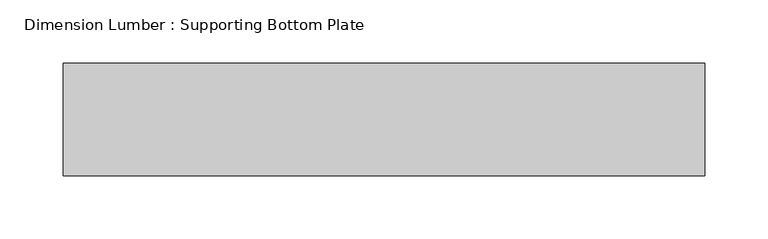
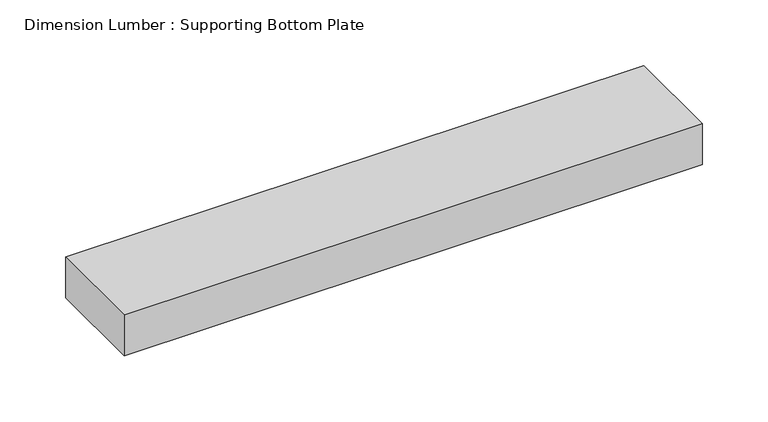
"""IFC4 building model written with IfcOpenShell, lengths in millimetres: beam geometry, Dimension Lumber : Supporting Bottom Plate."""

from ifc_helpers import new_model, si_unit, frame, origin, place, context, project, spatial, polyline, outline, extrude, source, transform, mapped, element, save


def dimension_lumber_supporting_bottom_plate_bde2bea7(model_context):
    return source(origin(), model_context, "Body", "SweptSolid", [
        extrude(outline(polyline([(-1203.025, 44.45), (-695.625, 44.45), (-695.625, -44.45), (-1203.025, -44.45), (-1203.025, 44.45)])), frame((0.0, 0.0, -19.05), z_axis=(0.0, 0.0, 1.0), x_axis=(1.0, 0.0, 0.0)), (0.0, 0.0, 1.0), 38.1),
    ])


if __name__ == "__main__":
    model = new_model("IFC4")
    model_context = context("Model", 3, world=origin())
    ifc_project = project(units=[si_unit("LENGTHUNIT", "METRE", prefix="MILLI")], contexts=[model_context])
    site = spatial("IfcSite", under=ifc_project)
    building = spatial("IfcBuilding", under=site)
    placement = place(None, origin())
    dimension_lumber_supporting_bottom_plate_shape = dimension_lumber_supporting_bottom_plate_bde2bea7(model_context)
    element("IfcBeam", 1, ObjectType="Dimension Lumber : Supporting Bottom Plate", at=placement, inside=building, context=model_context, shape_type="MappedRepresentation", body=[
        mapped(dimension_lumber_supporting_bottom_plate_shape, transform((0.0, 0.0, 0.0), x_axis=(1.0, 0.0, 0.0), y_axis=(0.0, 1.0, 0.0), z_axis=(0.0, 0.0, 1.0))),
    ])
    save(model, "model.ifc")

# Revit data of these elements
# Type "Dimension Lumber : Supporting Bottom Plate"
#   Assembly Code = "B10"
#   A = 0.0364583 SF
#   Length [instance default] = 5' - 0"
#   b = 0' - 3 1/2"
#   d = 0' - 1 1/2"
#   Structural Material [instance default] = Softwood, Lumber
# Element 1 (IfcBeam, "Dimension Lumber : Supporting Bottom Plate")
#   Structural Material = Douglas Fir #2
#   Materials on its faces: "Douglas Fir #2"
# Materials
#   "Softwood, Lumber": class "Wood", colour RGB 223 192 134, transparency 0, Description = "Pinus Echinata", Cost = 0
#   "Douglas Fir #2": class "Wood", colour RGB 223 192 134, transparency 0, Description = "Pinus Echinata", Cost = 0
